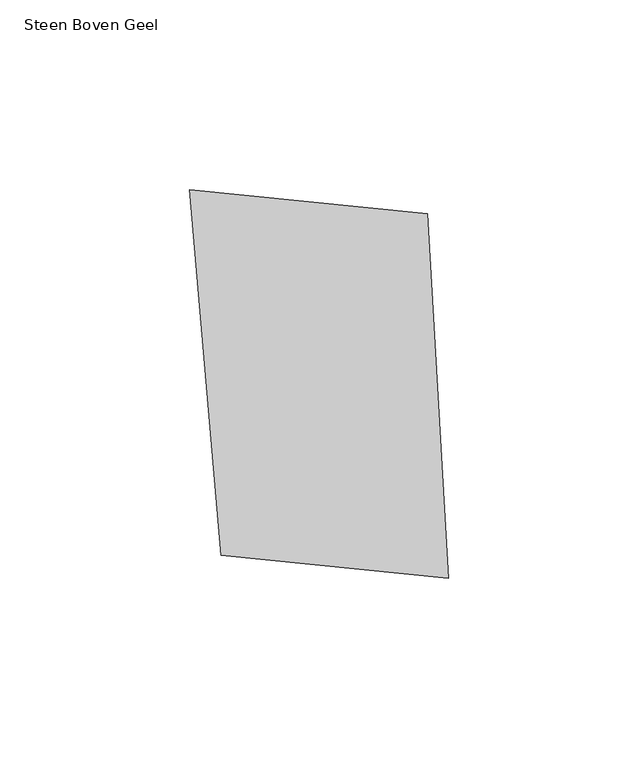
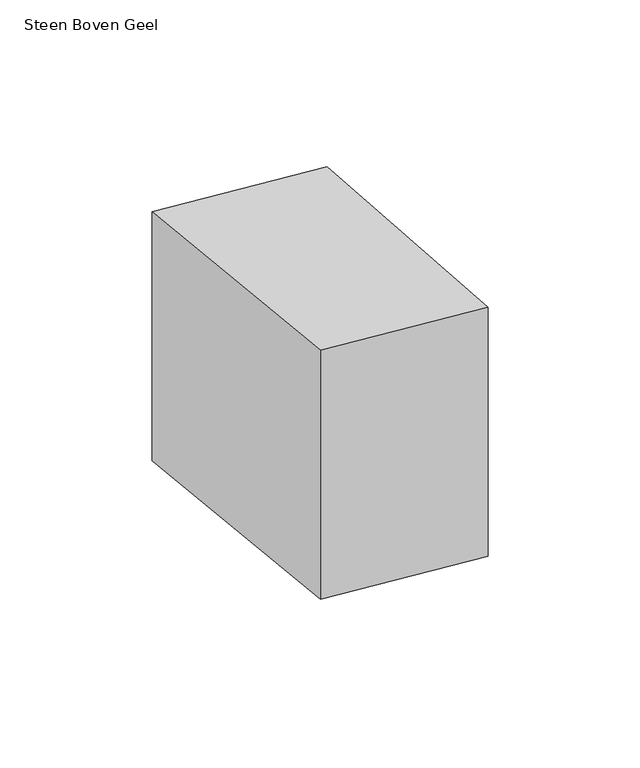
"""IFC4 building model written with IfcOpenShell, lengths in millimetres: proxy geometry, 00_GMA_steen_versie_4 : Steen Boven Geel."""

from ifc_helpers import new_model, si_unit, origin, origin_with_axes, place, context, project, spatial, polyline, outline, extrude, source, transform, mapped, element, save


def steen_boven_geel_b89bf64f(model_context):
    return source(origin(), model_context, "Body", "SweptSolid", [
        extrude(outline(polyline([(97.6463821, 119.6598354), (103.2216074, 23.5355691), (43.2360964, 29.6219847), (34.8938868, 126.0490883), (97.6463821, 119.6598354)])), origin_with_axes(), (0.0, 0.0, 1.0), 100.0),
    ])


if __name__ == "__main__":
    model = new_model("IFC4")
    model_context = context("Model", 3, world=origin())
    ifc_project = project(units=[si_unit("LENGTHUNIT", "METRE", prefix="MILLI")], contexts=[model_context])
    site = spatial("IfcSite", under=ifc_project)
    building = spatial("IfcBuilding", under=site)
    placement = place(None, origin())
    steen_boven_geel_shape = steen_boven_geel_b89bf64f(model_context)
    element("IfcBuildingElementProxy", 1, Name="00_GMA_steen_versie_4 : Steen Boven Geel", ObjectType="00_GMA_steen_versie_4 : Steen Boven Geel", at=placement, inside=building, context=model_context, shape_type="MappedRepresentation", body=[
        mapped(steen_boven_geel_shape, transform((0.0, 0.0, 0.0), x_axis=(1.0, 0.0, 0.0), y_axis=(0.0, 1.0, 0.0), z_axis=(0.0, 0.0, 1.0))),
    ])
    save(model, "model.ifc")

# Revit data of these elements
# Type "00_GMA_steen_versie_4 : Steen Boven Geel"
#   StootVoegHalfBoven [instance default] = 5 mm
#   StootVoegHalf [instance default] = 5 mm
#   StootVoegBreedteOnder = 10 mm
#   StootVoegBreedteBoven = 10 mm
#   Steendikte = 100 mm
#   LintVoegOnderHalf = 5 mm
#   LintVoegOnder = 10 mm
#   LintVoegBovenHalf = 0 mm
#   LintVoegBoven = 0 mm
#   materiaal = 21_steen_geel
#   MateriaalVoeg = none
#   Default Elevation = 0
# Element 1 (IfcBuildingElementProxy, "00_GMA_steen_versie_4 : Steen Boven Geel")
#   Materials on its faces: "21_steen_geel"
# Materials
#   "21_steen_geel": class "Unassigned", colour RGB 202 202 0, transparency 0, Cost = 0
